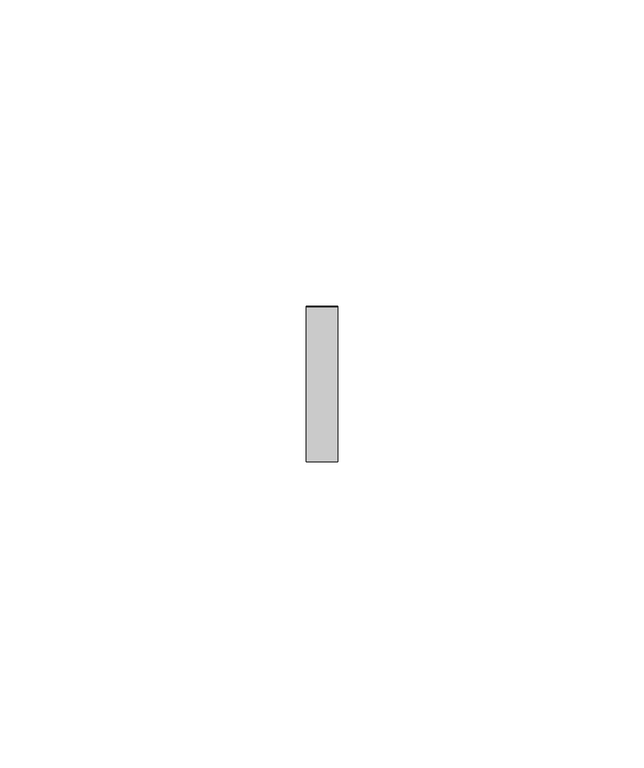
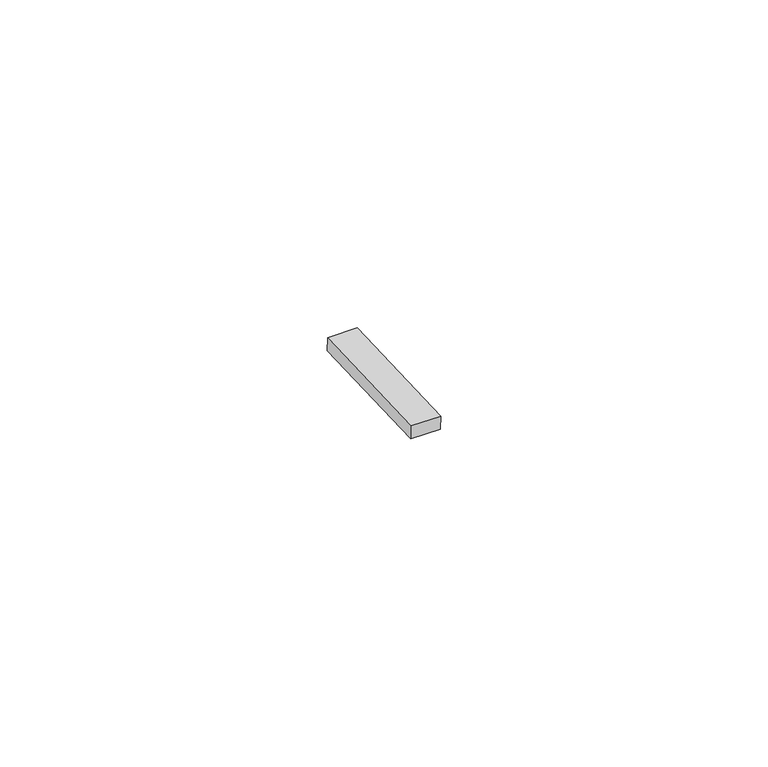
"""IFC4 building model written with IfcOpenShell, lengths in millimetres: proxy geometry, Inner panel:Inner panel:1:Inner panel:1 : Inner panel:Inner panel:300324:2:Inner panel:1:Inner panel:1 : Inner panel:Inner panel:300324:2 : Inner panel:Inner panel:1:Inner panel:1 : Inner panel:Inner panel:300324:300043:128 : Inner panel:Inner panel:1:Inner panel:1 : Inner panel:Inner panel:300324:2:Inner panel:1:Inner panel:1 : Inner panel:Inner panel:300324:2 : Inner panel:Inner panel:1:Inner panel:1 : Inner panel:Inner panel:300324:300043:308120."""

from ifc_helpers import new_model, si_unit, frame, origin, place, context, project, spatial, polyline, outline, extrude, source, transform, mapped, element, save


def generic_models_24aa216e(model_context):
    return source(origin(), model_context, "Body", "SweptSolid", [
        extrude(outline(polyline([(0.0, -25.3999999), (0.0, 0.0), (5.2138089, 0.0), (5.2138089, -25.3999999), (0.0, -25.3999999)])), frame((592310.995117, -577413.7950993, 4016.01903), z_axis=(0.0, -0.041630544712223896, 0.9991330730923502), x_axis=(-1.0, 0.0, 0.0)), (0.0, 0.0, 1.0), 2.4763745),
    ])


if __name__ == "__main__":
    model = new_model("IFC4")
    model_context = context("Model", 3, world=origin())
    ifc_project = project(units=[si_unit("LENGTHUNIT", "METRE", prefix="MILLI")], contexts=[model_context])
    site = spatial("IfcSite", under=ifc_project)
    building = spatial("IfcBuilding", under=site)
    placement = place(None, origin())
    generic_models_shape = generic_models_24aa216e(model_context)
    element("IfcBuildingElementProxy", 1, Name="Inner panel:Inner panel:1:Inner panel:1 : Inner panel:Inner panel:300324:2:Inner panel:1:Inner panel:1 : Inner panel:Inner panel:300324:2 : Inner panel:Inner panel:1:Inner panel:1 : Inner panel:Inner panel:300324:300043:128 : Inner panel:Inner panel:1:Inner panel:1 : Inner panel:Inner panel:300324:2:Inner panel:1:Inner panel:1 : Inner panel:Inner panel:300324:2 : Inner panel:Inner panel:1:Inner panel:1 : Inner panel:Inner panel:300324:300043:308120", ObjectType="Inner panel:Inner panel:1:Inner panel:1 : Inner panel:Inner panel:300324:2:Inner panel:1:Inner panel:1 : Inner panel:Inner panel:300324:2 : Inner panel:Inner panel:1:Inner panel:1 : Inner panel:Inner panel:300324:300043:128 : Inner panel:Inner panel:1:Inner panel:1 : Inner panel:Inner panel:300324:2:Inner panel:1:Inner panel:1 : Inner panel:Inner panel:300324:2 : Inner panel:Inner panel:1:Inner panel:1 : Inner panel:Inner panel:300324:300043:308120", at=placement, inside=building, context=model_context, shape_type="MappedRepresentation", body=[
        mapped(generic_models_shape, transform((0.0, 0.0, 0.0), x_axis=(1.0, 0.0, 0.0), y_axis=(0.0, 1.0, 0.0), z_axis=(0.0, 0.0, 1.0))),
    ])
    save(model, "model.ifc")

# Revit data of these elements
# Type "Inner panel:Inner panel:1:Inner panel:1 : Inner panel:Inner panel:300324:2:Inner panel:1:Inner panel:1 : Inner panel:Inner panel:300324:2 : Inner panel:Inner panel:1:Inner panel:1 : Inner panel:Inner panel:300324:300043:128 : Inner panel:Inner panel:1:Inner panel:1 : Inner panel:Inner panel:300324:2:Inner panel:1:Inner panel:1 : Inner panel:Inner panel:300324:2 : Inner panel:Inner panel:1:Inner panel:1 : Inner panel:Inner panel:300324:300043:308120"
#   NameOverride = "Inner panel:Inner panel:1:Inner panel:1 : Inner panel:Inner panel:300324:2:Inner panel:1:Inner panel:1 : Inner panel:Inner panel:300324:2 : Inner panel:Inner panel:1:Inner panel:1 : Inner panel:Inner panel:300324:300043:308120"
#   ObjectTypeOverride = "Inner panel:1:Inner panel:1 : Inner panel:Inner panel:300324:2 : Inner panel:Inner panel:1:Inner panel:1 : Inner panel:Inner panel:300324:300043"
#   Reference = "Inner panel"
#   Tag = "308120"
# Element 1 (IfcBuildingElementProxy, "Inner panel:Inner panel:1:Inner panel:1 : Inner panel:Inner panel:300324:2:Inner panel:1:Inner panel:1 : Inner panel:Inner panel:300324:2 : Inner panel:Inner panel:1:Inner panel:1 : Inner panel:Inner panel:300324:300043:128 : Inner panel:Inner panel:1:Inner panel:1 : Inner panel:Inner panel:300324:2:Inner panel:1:Inner panel:1 : Inner panel:Inner panel:300324:2 : Inner panel:Inner panel:1:Inner panel:1 : Inner panel:Inner panel:300324:300043:308120")
#   Materials on its faces: "AT CLIP - 1\" WIDE NON ABSORBENT, WEATHER-RESISTANT NEOPRENE/EPDM/SBR FOAM"
# Materials
#   "AT CLIP - 1\" WIDE NON ABSORBENT, WEATHER-RESISTANT NEOPRENE/EPDM/SBR FOAM": class "Generic", colour RGB 85 85 85, transparency 0, Cost = 0
